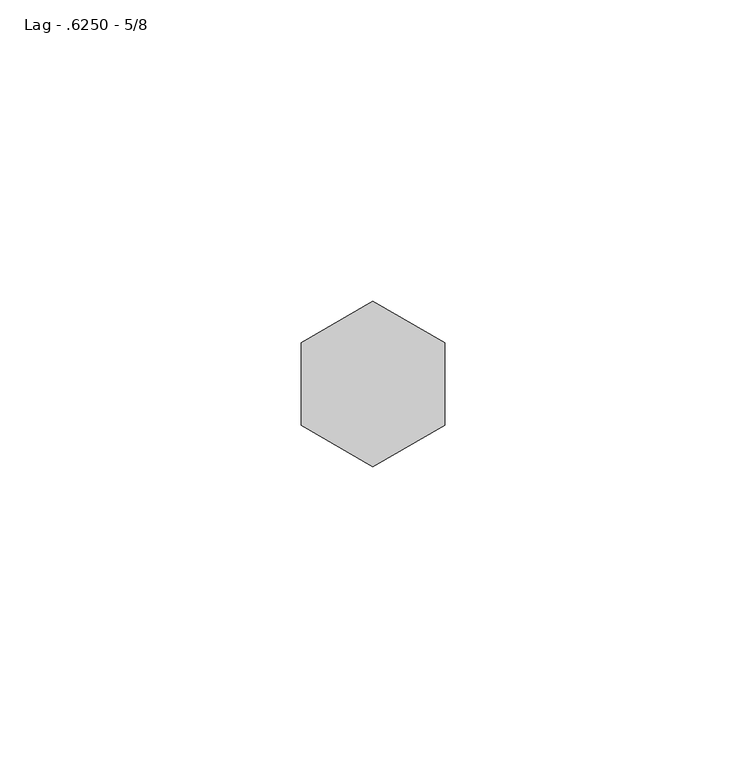
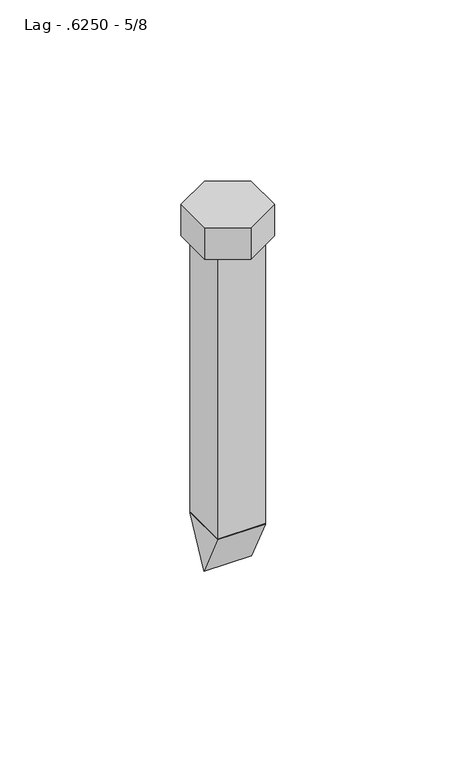
"""IFC4 building model written with IfcOpenShell, lengths in millimetres: fastener geometry, 060523 - W_P_C - Fastenings - Generic - SQUARE : Lag - .6250 - 5/8."""

from ifc_helpers import new_model, si_unit, frame, origin, origin_with_axes, place, context, project, spatial, polyline, outline, extrude, source, transform, mapped, element, save


def lag_6250_5_8_d0565a40(model_context):
    return source(origin(), model_context, "Body", "SweptSolid", [
        extrude(outline(polyline([(0.0, -117.871875), (-8.1359375, -101.6), (8.1359375, -101.6), (0.0, -117.871875)])), frame((-8.1359375, 0.0, 0.0), z_axis=(1.0, 0.0, 0.0), x_axis=(0.0, 1.0, 0.0)), (0.0, 0.0, 1.0), 16.271875),
        extrude(outline(polyline([(-11.90625, 6.8740766), (0.0, 13.7481533), (11.90625, 6.8740766), (11.90625, -6.8740766), (0.0, -13.7481533), (-11.90625, -6.8740766), (-11.90625, 6.8740766)])), origin_with_axes(), (0.0, 0.0, 1.0), 11.3109375),
        extrude(outline(polyline([(-8.1359375, 8.1359375), (8.1359375, 8.1359375), (8.1359375, -8.1359375), (-8.1359375, -8.1359375), (-8.1359375, 8.1359375)])), frame((0.0, 0.0, -101.6), z_axis=(0.0, 0.0, 1.0), x_axis=(1.0, 0.0, 0.0)), (0.0, 0.0, 1.0), 101.6),
    ])


if __name__ == "__main__":
    model = new_model("IFC4")
    model_context = context("Model", 3, world=origin())
    ifc_project = project(units=[si_unit("LENGTHUNIT", "METRE", prefix="MILLI")], contexts=[model_context])
    site = spatial("IfcSite", under=ifc_project)
    building = spatial("IfcBuilding", under=site)
    placement = place(None, origin())
    lag_6250_5_8_shape = lag_6250_5_8_d0565a40(model_context)
    element("IfcFastener", 1, ObjectType="060523 - W_P_C - Fastenings - Generic - SQUARE : Lag - .6250 - 5/8", at=placement, inside=building, context=model_context, shape_type="MappedRepresentation", body=[
        mapped(lag_6250_5_8_shape, transform((0.0, 0.0, 0.0), x_axis=(1.0, 0.0, 0.0), y_axis=(0.0, 1.0, 0.0), z_axis=(0.0, 0.0, 1.0))),
    ])
    save(model, "model.ifc")

# Revit data of these elements
# Type "060523 - W_P_C - Fastenings - Generic - SQUARE : Lag - .6250 - 5/8"
#   Washer_Thickness = 0' - 0 19/128"
#   Washer Radius = 0' - 0 49/64"
#   Washer Offset - Head = 0' - 0"
#   Washer Offset = 0' - 0"
#   Thickness_of_Substrate [instance default] = 0' - 1"
#   Side = 0' - 0.54199"
#   Radius = 0' - 0 41/128"
#   Length [instance default] = 0' - 4"
#   Head Size = 0' - 0 15/16"
#   Head Radius = 0' - 0 15/32"
#   Head Height = 0' - 0 57/128"
#   Double Diameter = 0' - 1 9/32"
#   Diameter = 0' - 0 41/64"
#   Default Elevation = 4' - 0"
#   Washer_Nut_Visibility = no
#   Washer_Head_Visibility = no
#   Round_Head_Visibility = no
#   Point Visibility = yes
#   Nut_Visibility = no
#   Hex_Head_Visiblilty = yes
#   Washer Material = none
#   Bolt Material (Size) = AT SILL - FASTENER AT 24" O.C.
# Element 1 (IfcFastener, "060523 - W_P_C - Fastenings - Generic - SQUARE : Lag - .6250 - 5/8")
#   Materials on its faces: "AT SILL - FASTENER AT 24\" O.C."
# Materials
#   "AT SILL - FASTENER AT 24\" O.C.": class "Generic", colour RGB 120 120 120, transparency 0, Cost = 0
